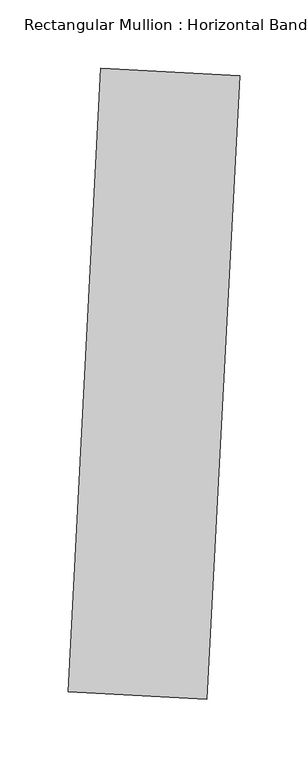
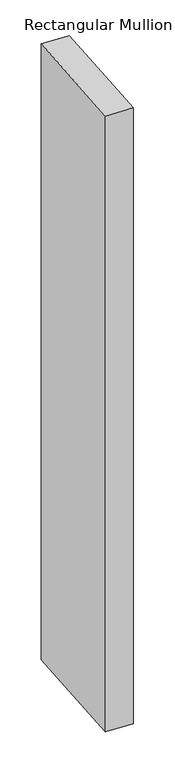
"""IFC4 building model written with IfcOpenShell, lengths in millimetres: member geometry, Rectangular Mullion : Horizontal Band."""

import ifcopenshell
import ifcopenshell.guid

model = None  # the IFC model being written
_history = None  # IfcOwnerHistory: only IFC2X3 demands one
_inside = {}  # id of a spatial element -> (the spatial element, [elements in it])
_under = {}  # id of a project, library or spatial element -> (it, [spatial elements below it])
_declared = {}  # id of a project -> (the project, [libraries it declares])
_typed = {}  # id of a type object -> (the type object, [elements of that type])
_made_of = {}  # id of a material, layer set ... -> (it, [elements and type objects made of it])


def new_model(schema):
    """Start an empty IFC model of exactly this schema.

    Asked for "IFC4X3", IfcOpenShell would pick the latest addendum, in which some entities
    have other attributes; the version numbers below select the first issue.
    IFC2X3 requires an IfcOwnerHistory on every rooted entity: one is made here for all.
    """
    global model, _history
    if schema == "IFC4X3":
        model = ifcopenshell.file(schema_version=(4, 3, 0, 0))
    else:
        model = ifcopenshell.file(schema=schema)
    _inside.clear()
    _under.clear()
    _declared.clear()
    _typed.clear()
    _made_of.clear()
    _history = None
    if model.schema == "IFC2X3":
        org = make("IfcOrganization", Name="unknown")
        user = make(
            "IfcPersonAndOrganization",
            ThePerson=make("IfcPerson", FamilyName="unknown"),
            TheOrganization=org,
        )
        app = make(
            "IfcApplication",
            ApplicationDeveloper=org,
            Version="unknown",
            ApplicationFullName="unknown",
            ApplicationIdentifier="unknown",
        )
        _history = make(
            "IfcOwnerHistory",
            OwningUser=user,
            OwningApplication=app,
            ChangeAction="ADDED",
            CreationDate=0,
        )
    return model


def make(cls, **values):
    """One entity of the class cls with the attributes given. An attribute that is None is left unset."""
    return model.create_entity(
        cls, **{name: value for name, value in values.items() if value is not None}
    )


def rooted(cls, **values):
    """An entity with a GlobalId (a new one), such as an element, a storey or a relation."""
    return make(cls, GlobalId=ifcopenshell.guid.new(), OwnerHistory=_history, **values)


def si_unit(unit_type, name, prefix=None):
    """IfcSIUnit, for example si_unit("LENGTHUNIT", "METRE", prefix="MILLI")."""
    return make("IfcSIUnit", UnitType=unit_type, Prefix=prefix, Name=name)


def assignment(units):
    """IfcUnitAssignment: the units of a project."""
    return None if units is None else make("IfcUnitAssignment", Units=units)


def point(xyz):
    """IfcCartesianPoint."""
    return None if xyz is None else make("IfcCartesianPoint", Coordinates=xyz)


def direction(xyz):
    """IfcDirection."""
    return None if xyz is None else make("IfcDirection", DirectionRatios=xyz)


def frame(location, z_axis=None, x_axis=None):
    """IfcAxis2Placement3D, a coordinate frame: its origin and axes. An axis left out is left unset."""
    return make(
        "IfcAxis2Placement3D",
        Location=point(location),
        Axis=direction(z_axis),
        RefDirection=direction(x_axis),
    )


def origin():
    """The frame at (0, 0, 0) with its axes left unset."""
    return frame((0.0, 0.0, 0.0))


def place(relative_to, where):
    """IfcLocalPlacement: puts the frame where relative to a parent placement (None: the world)."""
    return make(
        "IfcLocalPlacement", PlacementRelTo=relative_to, RelativePlacement=where
    )


def context(
    kind, dimensions, precision=None, world=None, true_north=None, identifier=None
):
    """IfcGeometricRepresentationContext, for example the 3D "Model" context."""
    return make(
        "IfcGeometricRepresentationContext",
        ContextIdentifier=identifier,
        ContextType=kind,
        CoordinateSpaceDimension=dimensions,
        Precision=precision,
        WorldCoordinateSystem=world,
        TrueNorth=true_north,
    )


def project(units=None, contexts=None):
    """IfcProject with its units and contexts."""
    return rooted(
        "IfcProject",
        Name="project",
        RepresentationContexts=contexts,
        UnitsInContext=assignment(units),
    )


def spatial(cls, under=None, at=None, **own):
    """A site, building, storey or space (cls), placed at a placement, below another one or the project."""
    s = rooted(cls, ObjectPlacement=at, **own)
    if under is not None:
        _under.setdefault(under.id(), (under, []))[1].append(s)
    return s


def polyline(points):
    """IfcPolyline through the points."""
    return make("IfcPolyline", Points=[point(p) for p in points])


def outline(outer, holes=None, kind="AREA"):
    """IfcArbitraryClosedProfileDef: a profile drawn as a closed curve; with holes, ...WithVoids."""
    if holes is None:
        return make("IfcArbitraryClosedProfileDef", ProfileType=kind, OuterCurve=outer)
    return make(
        "IfcArbitraryProfileDefWithVoids",
        ProfileType=kind,
        OuterCurve=outer,
        InnerCurves=holes,
    )


def extrude(swept, where, along, depth):
    """IfcExtrudedAreaSolid: the profile swept, set in the frame where, extruded along a direction by depth."""
    return make(
        "IfcExtrudedAreaSolid",
        SweptArea=swept,
        Position=where,
        ExtrudedDirection=direction(along),
        Depth=depth,
    )


def shape(context_of_items, identifier, shape_type, items):
    """IfcShapeRepresentation: the items that make up one representation, for example the "Body"."""
    return make(
        "IfcShapeRepresentation",
        ContextOfItems=context_of_items,
        RepresentationIdentifier=identifier,
        RepresentationType=shape_type,
        Items=items,
    )


def source(mapping_origin, context_of_items, identifier, shape_type, items):
    """IfcRepresentationMap: a shape defined once, which mapped items show again and again."""
    return make(
        "IfcRepresentationMap",
        MappingOrigin=mapping_origin,
        MappedRepresentation=shape(context_of_items, identifier, shape_type, items),
    )


def transform(
    local_origin,
    x_axis=None,
    y_axis=None,
    z_axis=None,
    scale=None,
    scale2=None,
    scale3=None,
    uniform=True,
):
    """IfcCartesianTransformationOperator3D, or its non-uniform kind. x_axis, y_axis, z_axis: its Axis1, 2, 3."""
    if uniform:
        return make(
            "IfcCartesianTransformationOperator3D",
            Axis1=direction(x_axis),
            Axis2=direction(y_axis),
            LocalOrigin=point(local_origin),
            Scale=scale,
            Axis3=direction(z_axis),
        )
    return make(
        "IfcCartesianTransformationOperator3DnonUniform",
        Axis1=direction(x_axis),
        Axis2=direction(y_axis),
        LocalOrigin=point(local_origin),
        Scale=scale,
        Axis3=direction(z_axis),
        Scale2=scale2,
        Scale3=scale3,
    )


def mapped(mapping_source, mapping_target):
    """IfcMappedItem: shows the shape of a source again, moved by a transform."""
    return make(
        "IfcMappedItem", MappingSource=mapping_source, MappingTarget=mapping_target
    )


def made_of(thing, what):
    """Note that an element or type object is made of a material, layer set ...; save() writes the relation."""
    if what is not None:
        _made_of.setdefault(what.id(), (what, []))[1].append(thing)
    return thing


def element(
    cls,
    number,
    at=None,
    inside=None,
    cuts=None,
    type_object=None,
    material=None,
    context=None,
    identifier="Body",
    shape_type=None,
    held_by="IfcProductDefinitionShape",
    body=None,
    shapes=None,
    **own,
):
    """One element of the class cls, such as IfcWall. Its Tag is "e" and its number.

    at: its placement. inside: the storey or other place that contains it. cuts: it is an
    opening in that element (IfcRelVoidsElement). A single representation is given by context,
    identifier, shape_type and body (its items); several are given by shapes. held_by: the class
    of the entity that holds the representations. save() writes the other relations.
    """
    e = rooted(cls, Tag="e%d" % number, ObjectPlacement=at, **own)
    if body is not None:
        shapes = [shape(context, identifier, shape_type, body)]
    if shapes is not None:
        e.Representation = make(held_by, Representations=shapes)
    if inside is not None:
        _inside.setdefault(inside.id(), (inside, []))[1].append(e)
    if cuts is not None:
        rooted(
            "IfcRelVoidsElement", RelatingBuildingElement=cuts, RelatedOpeningElement=e
        )
    if type_object is not None:
        _typed.setdefault(type_object.id(), (type_object, []))[1].append(e)
    return made_of(e, material)


def aggregate(whole, parts):
    """IfcRelAggregates: a whole, such as a stair, and the parts it consists of."""
    return rooted("IfcRelAggregates", RelatingObject=whole, RelatedObjects=parts)


def save(model, path):
    """Write the relations noted so far, then the file.

    IfcRelAggregates (storeys below a building ...), IfcRelContainedInSpatialStructure (elements
    in a storey), IfcRelDefinesByType, IfcRelAssociatesMaterial and IfcRelDeclares: one each for
    every whole, place, type object, material and project.
    """
    for whole, parts in _under.values():
        aggregate(whole, parts)
    for where, things in _inside.values():
        rooted(
            "IfcRelContainedInSpatialStructure",
            RelatedElements=things,
            RelatingStructure=where,
        )
    for kind, things in _typed.values():
        rooted("IfcRelDefinesByType", RelatedObjects=things, RelatingType=kind)
    for what, things in _made_of.values():
        rooted("IfcRelAssociatesMaterial", RelatedObjects=things, RelatingMaterial=what)
    for by, libraries in _declared.values():
        rooted("IfcRelDeclares", RelatingContext=by, RelatedDefinitions=libraries)
    model.write(path)


def rectangular_mullion_horizontal_band_9c283acf(model_context):
    return source(origin(), model_context, "Body", "SweptSolid", [
        extrude(outline(polyline([(62.69438, 301.8280451), (38.7663808, -154.7453782), (-62.69438, -149.4280451), (-38.7663808, 307.1453782), (62.69438, 301.8280451)])), frame((0.0, 0.0, -2437.4403502), z_axis=(0.0, 0.0, 1.0), x_axis=(1.0, 0.0, 0.0)), (0.0, 0.0, 1.0), 2437.4403502),
    ])


if __name__ == "__main__":
    model = new_model("IFC4")
    model_context = context("Model", 3, world=origin())
    ifc_project = project(units=[si_unit("LENGTHUNIT", "METRE", prefix="MILLI")], contexts=[model_context])
    site = spatial("IfcSite", under=ifc_project)
    building = spatial("IfcBuilding", under=site)
    placement = place(None, origin())
    rectangular_mullion_horizontal_band_shape = rectangular_mullion_horizontal_band_9c283acf(model_context)
    element("IfcMember", 1, ObjectType="Rectangular Mullion : Horizontal Band", at=placement, inside=building, context=model_context, shape_type="MappedRepresentation", body=[
        mapped(rectangular_mullion_horizontal_band_shape, transform((0.0, 0.0, 0.0), x_axis=(1.0, 0.0, 0.0), y_axis=(0.0, 1.0, 0.0), z_axis=(0.0, 0.0, 1.0))),
    ])
    save(model, "model.ifc")

# Revit data of these elements
# Type "Rectangular Mullion : Horizontal Band"
#   built-in parameter 1007351 = 0.25 (stored number, unit not read)
#   built-in parameter 1007304 = 1.5 (stored number, unit not read)
#   built-in parameter 1007301 = 0.166667 (stored number, unit not read)
#   built-in parameter 1007300 = 0.166667 (stored number, unit not read)
# Element 1 (IfcMember, "Rectangular Mullion : Horizontal Band")
#   Materials on its faces: "Aluminum"
# Materials
#   "Aluminum": class "Metal", colour RGB 247 247 247, transparency 0, Description = "Aluminum 6061", Cost = 0
